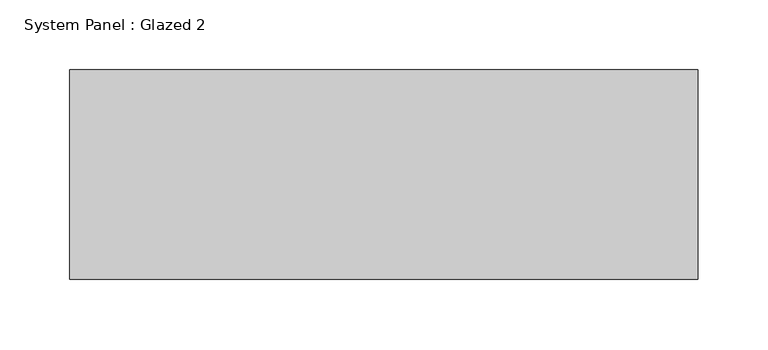
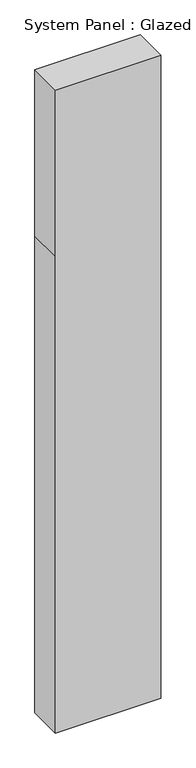
"""IFC4 building model written with IfcOpenShell, lengths in millimetres: plate geometry, System Panel : Glazed 2."""

from ifc_helpers import new_model, si_unit, frame, origin, place, context, project, spatial, polyline, outline, extrude, source, transform, mapped, element, save


def system_panel_glazed_2_4ff4bf1d(model_context):
    return source(origin(), model_context, "Body", "SweptSolid", [
        extrude(outline(polyline([(0.0, -225.0), (0.0, 225.0), (2150.0, 225.0), (2900.0, 225.0), (2900.0, -225.0), (2150.0, -225.0), (0.0, -225.0)])), frame((0.0, -75.0, 0.0), z_axis=(0.0, 1.0, 0.0), x_axis=(0.0, 0.0, 1.0)), (0.0, 0.0, 1.0), 150.0),
    ])


if __name__ == "__main__":
    model = new_model("IFC4")
    model_context = context("Model", 3, world=origin())
    ifc_project = project(units=[si_unit("LENGTHUNIT", "METRE", prefix="MILLI")], contexts=[model_context])
    site = spatial("IfcSite", under=ifc_project)
    building = spatial("IfcBuilding", under=site)
    placement = place(None, origin())
    system_panel_glazed_2_shape = system_panel_glazed_2_4ff4bf1d(model_context)
    element("IfcPlate", 1, ObjectType="System Panel : Glazed 2", at=placement, inside=building, context=model_context, shape_type="MappedRepresentation", body=[
        mapped(system_panel_glazed_2_shape, transform((0.0, 0.0, 0.0), x_axis=(1.0, 0.0, 0.0), y_axis=(0.0, 1.0, 0.0), z_axis=(0.0, 0.0, 1.0))),
    ])
    save(model, "model.ifc")

# Revit data of these elements
# Type "System Panel : Glazed 2"
#   COBie.Type = no
# Element 1 (IfcPlate, "System Panel : Glazed 2")
#   Materials on its faces: "Glass"
# Materials
#   "Glass": class "Glass", colour RGB 0 128 192, transparency 0.75, Description = "Soda Lime Glass", Cost = 0
